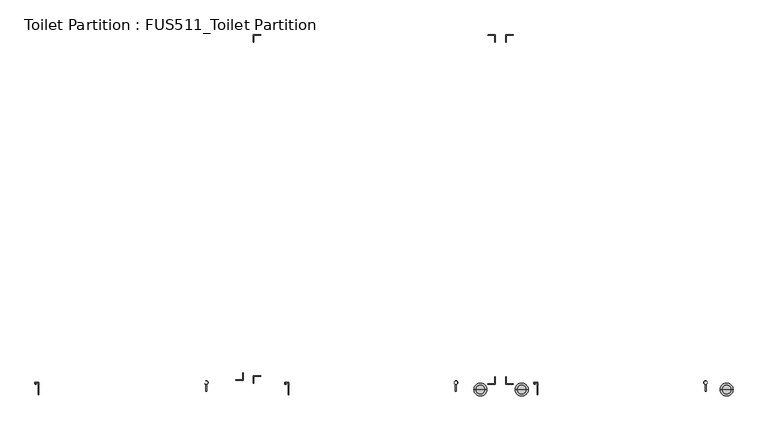
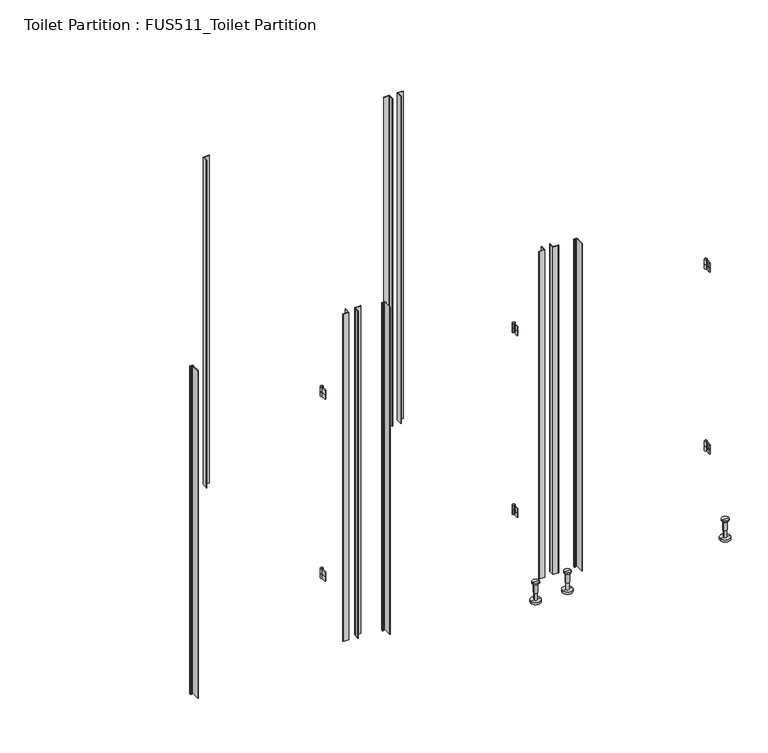
"""IFC4 building model written with IfcOpenShell, lengths in millimetres: furniture geometry, Toilet Partition : FUS511_Toilet Partition."""

import ifcopenshell
import ifcopenshell.guid

model = None  # the IFC model being written
_history = None  # IfcOwnerHistory: only IFC2X3 demands one
_inside = {}  # id of a spatial element -> (the spatial element, [elements in it])
_under = {}  # id of a project, library or spatial element -> (it, [spatial elements below it])
_declared = {}  # id of a project -> (the project, [libraries it declares])
_typed = {}  # id of a type object -> (the type object, [elements of that type])
_made_of = {}  # id of a material, layer set ... -> (it, [elements and type objects made of it])


def new_model(schema):
    """Start an empty IFC model of exactly this schema.

    Asked for "IFC4X3", IfcOpenShell would pick the latest addendum, in which some entities
    have other attributes; the version numbers below select the first issue.
    IFC2X3 requires an IfcOwnerHistory on every rooted entity: one is made here for all.
    """
    global model, _history
    if schema == "IFC4X3":
        model = ifcopenshell.file(schema_version=(4, 3, 0, 0))
    else:
        model = ifcopenshell.file(schema=schema)
    _inside.clear()
    _under.clear()
    _declared.clear()
    _typed.clear()
    _made_of.clear()
    _history = None
    if model.schema == "IFC2X3":
        org = make("IfcOrganization", Name="unknown")
        user = make(
            "IfcPersonAndOrganization",
            ThePerson=make("IfcPerson", FamilyName="unknown"),
            TheOrganization=org,
        )
        app = make(
            "IfcApplication",
            ApplicationDeveloper=org,
            Version="unknown",
            ApplicationFullName="unknown",
            ApplicationIdentifier="unknown",
        )
        _history = make(
            "IfcOwnerHistory",
            OwningUser=user,
            OwningApplication=app,
            ChangeAction="ADDED",
            CreationDate=0,
        )
    return model


def make(cls, **values):
    """One entity of the class cls with the attributes given. An attribute that is None is left unset."""
    return model.create_entity(
        cls, **{name: value for name, value in values.items() if value is not None}
    )


def rooted(cls, **values):
    """An entity with a GlobalId (a new one), such as an element, a storey or a relation."""
    return make(cls, GlobalId=ifcopenshell.guid.new(), OwnerHistory=_history, **values)


def si_unit(unit_type, name, prefix=None):
    """IfcSIUnit, for example si_unit("LENGTHUNIT", "METRE", prefix="MILLI")."""
    return make("IfcSIUnit", UnitType=unit_type, Prefix=prefix, Name=name)


def assignment(units):
    """IfcUnitAssignment: the units of a project."""
    return None if units is None else make("IfcUnitAssignment", Units=units)


def point(xyz):
    """IfcCartesianPoint."""
    return None if xyz is None else make("IfcCartesianPoint", Coordinates=xyz)


def direction(xyz):
    """IfcDirection."""
    return None if xyz is None else make("IfcDirection", DirectionRatios=xyz)


def frame(location, z_axis=None, x_axis=None):
    """IfcAxis2Placement3D, a coordinate frame: its origin and axes. An axis left out is left unset."""
    return make(
        "IfcAxis2Placement3D",
        Location=point(location),
        Axis=direction(z_axis),
        RefDirection=direction(x_axis),
    )


def frame_2d(location, x_axis=None):
    """IfcAxis2Placement2D, a coordinate frame in the plane: its origin and x axis."""
    return make(
        "IfcAxis2Placement2D", Location=point(location), RefDirection=direction(x_axis)
    )


def origin():
    """The frame at (0, 0, 0) with its axes left unset."""
    return frame((0.0, 0.0, 0.0))


def place(relative_to, where):
    """IfcLocalPlacement: puts the frame where relative to a parent placement (None: the world)."""
    return make(
        "IfcLocalPlacement", PlacementRelTo=relative_to, RelativePlacement=where
    )


def context(
    kind, dimensions, precision=None, world=None, true_north=None, identifier=None
):
    """IfcGeometricRepresentationContext, for example the 3D "Model" context."""
    return make(
        "IfcGeometricRepresentationContext",
        ContextIdentifier=identifier,
        ContextType=kind,
        CoordinateSpaceDimension=dimensions,
        Precision=precision,
        WorldCoordinateSystem=world,
        TrueNorth=true_north,
    )


def project(units=None, contexts=None):
    """IfcProject with its units and contexts."""
    return rooted(
        "IfcProject",
        Name="project",
        RepresentationContexts=contexts,
        UnitsInContext=assignment(units),
    )


def spatial(cls, under=None, at=None, **own):
    """A site, building, storey or space (cls), placed at a placement, below another one or the project."""
    s = rooted(cls, ObjectPlacement=at, **own)
    if under is not None:
        _under.setdefault(under.id(), (under, []))[1].append(s)
    return s


def polyline(points):
    """IfcPolyline through the points."""
    return make("IfcPolyline", Points=[point(p) for p in points])


def circle_curve(where, radius):
    """IfcCircle in the frame where."""
    return make("IfcCircle", Position=where, Radius=radius)


def trimmed(basis, trim1, trim2, sense, master):
    """IfcTrimmedCurve: the piece of a basis curve between two trims."""
    return make(
        "IfcTrimmedCurve",
        BasisCurve=basis,
        Trim1=trim1,
        Trim2=trim2,
        SenseAgreement=sense,
        MasterRepresentation=master,
    )


def segment(curve, same_sense, transition):
    """IfcCompositeCurveSegment."""
    return make(
        "IfcCompositeCurveSegment",
        Transition=transition,
        SameSense=same_sense,
        ParentCurve=curve,
    )


def composite_curve(segments, self_intersect=None):
    """IfcCompositeCurve: segments joined end to end."""
    return make("IfcCompositeCurve", Segments=segments, SelfIntersect=self_intersect)


def outline(outer, holes=None, kind="AREA"):
    """IfcArbitraryClosedProfileDef: a profile drawn as a closed curve; with holes, ...WithVoids."""
    if holes is None:
        return make("IfcArbitraryClosedProfileDef", ProfileType=kind, OuterCurve=outer)
    return make(
        "IfcArbitraryProfileDefWithVoids",
        ProfileType=kind,
        OuterCurve=outer,
        InnerCurves=holes,
    )


def extrude(swept, where, along, depth):
    """IfcExtrudedAreaSolid: the profile swept, set in the frame where, extruded along a direction by depth."""
    return make(
        "IfcExtrudedAreaSolid",
        SweptArea=swept,
        Position=where,
        ExtrudedDirection=direction(along),
        Depth=depth,
    )


def shape(context_of_items, identifier, shape_type, items):
    """IfcShapeRepresentation: the items that make up one representation, for example the "Body"."""
    return make(
        "IfcShapeRepresentation",
        ContextOfItems=context_of_items,
        RepresentationIdentifier=identifier,
        RepresentationType=shape_type,
        Items=items,
    )


def source(mapping_origin, context_of_items, identifier, shape_type, items):
    """IfcRepresentationMap: a shape defined once, which mapped items show again and again."""
    return make(
        "IfcRepresentationMap",
        MappingOrigin=mapping_origin,
        MappedRepresentation=shape(context_of_items, identifier, shape_type, items),
    )


def transform(
    local_origin,
    x_axis=None,
    y_axis=None,
    z_axis=None,
    scale=None,
    scale2=None,
    scale3=None,
    uniform=True,
):
    """IfcCartesianTransformationOperator3D, or its non-uniform kind. x_axis, y_axis, z_axis: its Axis1, 2, 3."""
    if uniform:
        return make(
            "IfcCartesianTransformationOperator3D",
            Axis1=direction(x_axis),
            Axis2=direction(y_axis),
            LocalOrigin=point(local_origin),
            Scale=scale,
            Axis3=direction(z_axis),
        )
    return make(
        "IfcCartesianTransformationOperator3DnonUniform",
        Axis1=direction(x_axis),
        Axis2=direction(y_axis),
        LocalOrigin=point(local_origin),
        Scale=scale,
        Axis3=direction(z_axis),
        Scale2=scale2,
        Scale3=scale3,
    )


def mapped(mapping_source, mapping_target):
    """IfcMappedItem: shows the shape of a source again, moved by a transform."""
    return make(
        "IfcMappedItem", MappingSource=mapping_source, MappingTarget=mapping_target
    )


def made_of(thing, what):
    """Note that an element or type object is made of a material, layer set ...; save() writes the relation."""
    if what is not None:
        _made_of.setdefault(what.id(), (what, []))[1].append(thing)
    return thing


def element(
    cls,
    number,
    at=None,
    inside=None,
    cuts=None,
    type_object=None,
    material=None,
    context=None,
    identifier="Body",
    shape_type=None,
    held_by="IfcProductDefinitionShape",
    body=None,
    shapes=None,
    **own,
):
    """One element of the class cls, such as IfcWall. Its Tag is "e" and its number.

    at: its placement. inside: the storey or other place that contains it. cuts: it is an
    opening in that element (IfcRelVoidsElement). A single representation is given by context,
    identifier, shape_type and body (its items); several are given by shapes. held_by: the class
    of the entity that holds the representations. save() writes the other relations.
    """
    e = rooted(cls, Tag="e%d" % number, ObjectPlacement=at, **own)
    if body is not None:
        shapes = [shape(context, identifier, shape_type, body)]
    if shapes is not None:
        e.Representation = make(held_by, Representations=shapes)
    if inside is not None:
        _inside.setdefault(inside.id(), (inside, []))[1].append(e)
    if cuts is not None:
        rooted(
            "IfcRelVoidsElement", RelatingBuildingElement=cuts, RelatedOpeningElement=e
        )
    if type_object is not None:
        _typed.setdefault(type_object.id(), (type_object, []))[1].append(e)
    return made_of(e, material)


def aggregate(whole, parts):
    """IfcRelAggregates: a whole, such as a stair, and the parts it consists of."""
    return rooted("IfcRelAggregates", RelatingObject=whole, RelatedObjects=parts)


def save(model, path):
    """Write the relations noted so far, then the file.

    IfcRelAggregates (storeys below a building ...), IfcRelContainedInSpatialStructure (elements
    in a storey), IfcRelDefinesByType, IfcRelAssociatesMaterial and IfcRelDeclares: one each for
    every whole, place, type object, material and project.
    """
    for whole, parts in _under.values():
        aggregate(whole, parts)
    for where, things in _inside.values():
        rooted(
            "IfcRelContainedInSpatialStructure",
            RelatedElements=things,
            RelatingStructure=where,
        )
    for kind, things in _typed.values():
        rooted("IfcRelDefinesByType", RelatedObjects=things, RelatingType=kind)
    for what, things in _made_of.values():
        rooted("IfcRelAssociatesMaterial", RelatedObjects=things, RelatingMaterial=what)
    for by, libraries in _declared.values():
        rooted("IfcRelDeclares", RelatingContext=by, RelatedDefinitions=libraries)
    model.write(path)


def plane_surface(at):
    """IfcPlane: the flat surface through the origin of the frame at, square to its z axis."""
    return make("IfcPlane", Position=at)


def cylinder_surface(at, radius):
    """IfcCylindricalSurface: all points at the distance radius from the z axis of the frame at."""
    return make("IfcCylindricalSurface", Position=at, Radius=radius)


def advanced_brep(points, edges, surfaces, faces):
    """IfcAdvancedBrep: a solid bounded by faces that lie on surfaces and meet in shared edges.

    An edge is (start, end): straight between two places in points (the first is 0);
    or (start, end, curve); or (start, end, curve, False) where it runs against its curve.
    A face is (place in surfaces, loops), or (place, loops, False) where it looks against
    its surface's normal. A loop lists edges by number (the first is 1), with a minus sign
    where the edge is run from its end to its start. The first loop is the outer one.
    """
    corners = [point(p) for p in points]
    vertices = [make("IfcVertexPoint", VertexGeometry=c) for c in corners]
    made = []
    for start, end, *more in edges:
        made.append(
            make(
                "IfcEdgeCurve",
                EdgeStart=vertices[start],
                EdgeEnd=vertices[end],
                EdgeGeometry=more[0] if more else make("IfcPolyline", Points=[corners[start], corners[end]]),
                SameSense=more[1] if len(more) > 1 else True,
            )
        )
    hull = []
    for where, loops, *sense in faces:
        bounds = []
        for j, loop in enumerate(loops):
            ring = [make("IfcOrientedEdge", EdgeElement=made[abs(k) - 1], Orientation=k > 0) for k in loop]
            bounds.append(
                make(
                    "IfcFaceOuterBound" if j == 0 else "IfcFaceBound",
                    Bound=make("IfcEdgeLoop", EdgeList=ring),
                    Orientation=True,
                )
            )
        hull.append(make("IfcAdvancedFace", Bounds=bounds, FaceSurface=surfaces[where], SameSense=sense[0] if sense else True))
    return make("IfcAdvancedBrep", Outer=make("IfcClosedShell", CfsFaces=hull))


def toilet_partition_fus511_toilet_partition_2a8fb3a8(model_context):
    return source(origin(), model_context, "Body", "SolidModel", [
        extrude(outline(composite_curve([segment(trimmed(circle_curve(frame_2d((-483.6851629, 1892.2118377)), 1.0008364), [point((-483.6851629, 1893.2126742))], [point((-484.6859993, 1892.2118377))], True, "CARTESIAN"), True, "CONTINUOUS"), segment(polyline([(-484.6859993, 1892.2118377), (-484.6859993, 1865.1892547), (-485.6868357, 1865.1892547)]), True, "CONTINUOUS"), segment(trimmed(circle_curve(frame_2d((-485.6868357, 1866.1900911)), 1.0008364), [point((-485.6868357, 1865.1892547))], [point((-486.6876721, 1866.1900911))], False, "CARTESIAN"), True, "CONTINUOUS"), segment(polyline([(-486.6876721, 1866.1900911), (-486.6876721, 1895.214347), (-457.6634163, 1895.214347)]), True, "CONTINUOUS"), segment(trimmed(circle_curve(frame_2d((-457.6634163, 1894.2135106)), 1.0008364), [point((-457.6634163, 1895.214347))], [point((-456.6625798, 1894.2135106))], False, "CARTESIAN"), True, "CONTINUOUS"), segment(polyline([(-456.6625798, 1894.2135106), (-456.6625798, 1893.2126742), (-483.6851629, 1893.2126742)]), True, "CONTINUOUS")], self_intersect=False)), frame((0.0, 0.0, 100.0), z_axis=(0.0, 0.0, 1.0), x_axis=(1.0, 0.0, 0.0)), (0.0, 0.0, 1.0), 1800.0),
        extrude(outline(composite_curve([segment(polyline([(478.8769058, 1893.2126742), (451.8543227, 1893.2126742), (451.8543227, 1894.2135106)]), True, "CONTINUOUS"), segment(trimmed(circle_curve(frame_2d((452.8551591, 1894.2135106)), 1.0008364), [point((451.8543227, 1894.2135106))], [point((452.8551591, 1895.214347))], False, "CARTESIAN"), True, "CONTINUOUS"), segment(polyline([(452.8551591, 1895.214347), (481.879415, 1895.214347), (481.879415, 1866.1900911)]), True, "CONTINUOUS"), segment(trimmed(circle_curve(frame_2d((480.8785786, 1866.1900911)), 1.0008364), [point((481.879415, 1866.1900911))], [point((480.8785786, 1865.1892547))], False, "CARTESIAN"), True, "CONTINUOUS"), segment(polyline([(480.8785786, 1865.1892547), (479.8777422, 1865.1892547), (479.8777422, 1892.2118377)]), True, "CONTINUOUS"), segment(trimmed(circle_curve(frame_2d((478.8769058, 1892.2118377)), 1.0008364), [point((479.8777422, 1892.2118377))], [point((478.8769058, 1893.2126742))], True, "CARTESIAN"), True, "CONTINUOUS")], self_intersect=False)), frame((0.0, 0.0, 100.0), z_axis=(0.0, 0.0, 1.0), x_axis=(1.0, 0.0, 0.0)), (0.0, 0.0, 1.0), 1800.0),
        extrude(outline(composite_curve([segment(trimmed(circle_curve(frame_2d((525.8819242, 1892.2118377)), 1.0008364), [point((525.8819242, 1893.2126742))], [point((524.8810878, 1892.2118377))], True, "CARTESIAN"), True, "CONTINUOUS"), segment(polyline([(524.8810878, 1892.2118377), (524.8810878, 1865.1892547), (523.8802514, 1865.1892547)]), True, "CONTINUOUS"), segment(trimmed(circle_curve(frame_2d((523.8802514, 1866.1900911)), 1.0008364), [point((523.8802514, 1865.1892547))], [point((522.879415, 1866.1900911))], False, "CARTESIAN"), True, "CONTINUOUS"), segment(polyline([(522.879415, 1866.1900911), (522.879415, 1895.214347), (551.9036709, 1895.214347)]), True, "CONTINUOUS"), segment(trimmed(circle_curve(frame_2d((551.9036709, 1894.2135106)), 1.0008364), [point((551.9036709, 1895.214347))], [point((552.9045073, 1894.2135106))], False, "CARTESIAN"), True, "CONTINUOUS"), segment(polyline([(552.9045073, 1894.2135106), (552.9045073, 1893.2126742), (525.8819242, 1893.2126742)]), True, "CONTINUOUS")], self_intersect=False)), frame((0.0, 0.0, 100.0), z_axis=(0.0, 0.0, 1.0), x_axis=(1.0, 0.0, 0.0)), (0.0, 0.0, 1.0), 1800.0),
        extrude(outline(composite_curve([segment(trimmed(circle_curve(frame_2d((-530.6901814, 514.4572016)), 1.0008364), [point((-530.6901814, 513.4563652))], [point((-529.689345, 514.4572016))], True, "CARTESIAN"), True, "CONTINUOUS"), segment(polyline([(-529.689345, 514.4572016), (-529.689345, 541.4797847), (-528.6885085, 541.4797847)]), True, "CONTINUOUS"), segment(trimmed(circle_curve(frame_2d((-528.6885085, 540.4789483)), 1.0008364), [point((-528.6885085, 541.4797847))], [point((-527.6876721, 540.4789483))], False, "CARTESIAN"), True, "CONTINUOUS"), segment(polyline([(-527.6876721, 540.4789483), (-527.6876721, 511.4546924), (-556.711928, 511.4546924)]), True, "CONTINUOUS"), segment(trimmed(circle_curve(frame_2d((-556.711928, 512.4555288)), 1.0008364), [point((-556.711928, 511.4546924))], [point((-557.7127644, 512.4555288))], False, "CARTESIAN"), True, "CONTINUOUS"), segment(polyline([(-557.7127644, 512.4555288), (-557.7127644, 513.4563652), (-530.6901814, 513.4563652)]), True, "CONTINUOUS")], self_intersect=False)), frame((0.0, 0.0, 100.0), z_axis=(0.0, 0.0, 1.0), x_axis=(1.0, 0.0, 0.0)), (0.0, 0.0, 1.0), 1800.0),
        extrude(outline(composite_curve([segment(trimmed(circle_curve(frame_2d((-483.6851629, 527.0159753)), 1.0008364), [point((-483.6851629, 528.0168117))], [point((-484.6859993, 527.0159753))], True, "CARTESIAN"), True, "CONTINUOUS"), segment(polyline([(-484.6859993, 527.0159753), (-484.6859993, 499.9933923), (-485.6868357, 499.9933923)]), True, "CONTINUOUS"), segment(trimmed(circle_curve(frame_2d((-485.6868357, 500.9942287)), 1.0008364), [point((-485.6868357, 499.9933923))], [point((-486.6876721, 500.9942287))], False, "CARTESIAN"), True, "CONTINUOUS"), segment(polyline([(-486.6876721, 500.9942287), (-486.6876721, 530.0184846), (-457.6634163, 530.0184846)]), True, "CONTINUOUS"), segment(trimmed(circle_curve(frame_2d((-457.6634163, 529.0176481)), 1.0008364), [point((-457.6634163, 530.0184846))], [point((-456.6625798, 529.0176481))], False, "CARTESIAN"), True, "CONTINUOUS"), segment(polyline([(-456.6625798, 529.0176481), (-456.6625798, 528.0168117), (-483.6851629, 528.0168117)]), True, "CONTINUOUS")], self_intersect=False)), frame((0.0, 0.0, 100.0), z_axis=(0.0, 0.0, 1.0), x_axis=(1.0, 0.0, 0.0)), (0.0, 0.0, 1.0), 1800.0),
        extrude(outline(composite_curve([segment(trimmed(circle_curve(frame_2d((478.8769058, 498.2168562)), 1.0008364), [point((478.8769058, 497.2160198))], [point((479.8777422, 498.2168562))], True, "CARTESIAN"), True, "CONTINUOUS"), segment(polyline([(479.8777422, 498.2168562), (479.8777422, 525.2394393), (480.8785786, 525.2394393)]), True, "CONTINUOUS"), segment(trimmed(circle_curve(frame_2d((480.8785786, 524.2386029)), 1.0008364), [point((480.8785786, 525.2394393))], [point((481.879415, 524.2386029))], False, "CARTESIAN"), True, "CONTINUOUS"), segment(polyline([(481.879415, 524.2386029), (481.879415, 495.214347), (452.8551591, 495.214347)]), True, "CONTINUOUS"), segment(trimmed(circle_curve(frame_2d((452.8551591, 496.2151834)), 1.0008364), [point((452.8551591, 495.214347))], [point((451.8543227, 496.2151834))], False, "CARTESIAN"), True, "CONTINUOUS"), segment(polyline([(451.8543227, 496.2151834), (451.8543227, 497.2160198), (478.8769058, 497.2160198)]), True, "CONTINUOUS")], self_intersect=False)), frame((0.0, 0.0, 100.0), z_axis=(0.0, 0.0, 1.0), x_axis=(1.0, 0.0, 0.0)), (0.0, 0.0, 1.0), 1800.0),
        extrude(outline(composite_curve([segment(polyline([(525.8819242, 497.2160198), (552.9045073, 497.2160198), (552.9045073, 496.2151834)]), True, "CONTINUOUS"), segment(trimmed(circle_curve(frame_2d((551.9036709, 496.2151834)), 1.0008364), [point((552.9045073, 496.2151834))], [point((551.9036709, 495.214347))], False, "CARTESIAN"), True, "CONTINUOUS"), segment(polyline([(551.9036709, 495.214347), (522.879415, 495.214347), (522.879415, 524.2386029)]), True, "CONTINUOUS"), segment(trimmed(circle_curve(frame_2d((523.8802514, 524.2386029)), 1.0008364), [point((522.879415, 524.2386029))], [point((523.8802514, 525.2394393))], False, "CARTESIAN"), True, "CONTINUOUS"), segment(polyline([(523.8802514, 525.2394393), (524.8810878, 525.2394393), (524.8810878, 498.2168562)]), True, "CONTINUOUS"), segment(trimmed(circle_curve(frame_2d((525.8819242, 498.2168562)), 1.0008364), [point((524.8810878, 498.2168562))], [point((525.8819242, 497.2160198))], True, "CARTESIAN"), True, "CONTINUOUS")], self_intersect=False)), frame((0.0, 0.0, 100.0), z_axis=(0.0, 0.0, 1.0), x_axis=(1.0, 0.0, 0.0)), (0.0, 0.0, 1.0), 1800.0),
        extrude(outline(composite_curve([segment(trimmed(circle_curve(frame_2d((1322.6156791, 502.2850056)), 7.0), [point((1320.6156791, 495.5768017))], [point((1324.6156791, 495.5768017))], False, "CARTESIAN"), True, "CONTINUOUS"), segment(polyline([(1324.6156791, 495.5768017), (1324.6156791, 467.7850056), (1320.6156791, 467.7850056), (1320.6156791, 495.5768017)]), True, "CONTINUOUS")], self_intersect=False), holes=[composite_curve([segment(trimmed(circle_curve(frame_2d((1322.6156791, 502.2850056)), 6.0), [point((1316.6156791, 502.2850056))], [point((1328.6156791, 502.2850056))], True, "CARTESIAN"), True, "CONTINUOUS"), segment(trimmed(circle_curve(frame_2d((1322.6156791, 502.2850056)), 6.0), [point((1328.6156791, 502.2850056))], [point((1316.6156791, 502.2850056))], True, "CARTESIAN"), True, "CONTINUOUS")], self_intersect=False)]), frame((0.0, 0.0, 1525.0), z_axis=(0.0, 0.0, 1.0), x_axis=(1.0, 0.0, 0.0)), (0.0, 0.0, 1.0), 25.0),
        extrude(outline(composite_curve([segment(trimmed(circle_curve(frame_2d((1322.6156791, 502.2850056)), 7.0), [point((1320.6156791, 495.5768017))], [point((1324.6156791, 495.5768017))], False, "CARTESIAN"), True, "CONTINUOUS"), segment(polyline([(1324.6156791, 495.5768017), (1324.6156791, 467.7850056), (1320.6156791, 467.7850056), (1320.6156791, 495.5768017)]), True, "CONTINUOUS")], self_intersect=False), holes=[composite_curve([segment(trimmed(circle_curve(frame_2d((1322.6156791, 502.2850056)), 6.0), [point((1316.6156791, 502.2850056))], [point((1328.6156791, 502.2850056))], True, "CARTESIAN"), True, "CONTINUOUS"), segment(trimmed(circle_curve(frame_2d((1322.6156791, 502.2850056)), 6.0), [point((1328.6156791, 502.2850056))], [point((1316.6156791, 502.2850056))], True, "CARTESIAN"), True, "CONTINUOUS")], self_intersect=False)]), frame((0.0, 0.0, 1500.0), z_axis=(0.0, 0.0, 1.0), x_axis=(1.0, 0.0, 0.0)), (0.0, 0.0, 1.0), 25.0),
        extrude(outline(composite_curve([segment(trimmed(circle_curve(frame_2d((323.7360042, 502.2850056)), 7.0), [point((321.7360042, 495.5768017))], [point((325.7360042, 495.5768017))], False, "CARTESIAN"), True, "CONTINUOUS"), segment(polyline([(325.7360042, 495.5768017), (325.7360042, 467.7850056), (321.7360042, 467.7850056), (321.7360042, 495.5768017)]), True, "CONTINUOUS")], self_intersect=False), holes=[composite_curve([segment(trimmed(circle_curve(frame_2d((323.7360042, 502.2850056)), 6.0), [point((317.7360042, 502.2850056))], [point((329.7360042, 502.2850056))], True, "CARTESIAN"), True, "CONTINUOUS"), segment(trimmed(circle_curve(frame_2d((323.7360042, 502.2850056)), 6.0), [point((329.7360042, 502.2850056))], [point((317.7360042, 502.2850056))], True, "CARTESIAN"), True, "CONTINUOUS")], self_intersect=False)]), frame((0.0, 0.0, 1525.0), z_axis=(0.0, 0.0, 1.0), x_axis=(1.0, 0.0, 0.0)), (0.0, 0.0, 1.0), 25.0),
        extrude(outline(composite_curve([segment(trimmed(circle_curve(frame_2d((323.7360042, 502.2850056)), 7.0), [point((321.7360042, 495.5768017))], [point((325.7360042, 495.5768017))], False, "CARTESIAN"), True, "CONTINUOUS"), segment(polyline([(325.7360042, 495.5768017), (325.7360042, 467.7850056), (321.7360042, 467.7850056), (321.7360042, 495.5768017)]), True, "CONTINUOUS")], self_intersect=False), holes=[composite_curve([segment(trimmed(circle_curve(frame_2d((323.7360042, 502.2850056)), 6.0), [point((317.7360042, 502.2850056))], [point((329.7360042, 502.2850056))], True, "CARTESIAN"), True, "CONTINUOUS"), segment(trimmed(circle_curve(frame_2d((323.7360042, 502.2850056)), 6.0), [point((329.7360042, 502.2850056))], [point((317.7360042, 502.2850056))], True, "CARTESIAN"), True, "CONTINUOUS")], self_intersect=False)]), frame((0.0, 0.0, 1500.0), z_axis=(0.0, 0.0, 1.0), x_axis=(1.0, 0.0, 0.0)), (0.0, 0.0, 1.0), 25.0),
        extrude(outline(composite_curve([segment(trimmed(circle_curve(frame_2d((-675.1953266, 502.2850056)), 7.0), [point((-677.1953266, 495.5768017))], [point((-673.1953266, 495.5768017))], False, "CARTESIAN"), True, "CONTINUOUS"), segment(polyline([(-673.1953266, 495.5768017), (-673.1953266, 467.7850056), (-677.1953266, 467.7850056), (-677.1953266, 495.5768017)]), True, "CONTINUOUS")], self_intersect=False), holes=[composite_curve([segment(trimmed(circle_curve(frame_2d((-675.1953266, 502.2850056)), 6.0), [point((-681.1953266, 502.2850056))], [point((-669.1953266, 502.2850056))], True, "CARTESIAN"), True, "CONTINUOUS"), segment(trimmed(circle_curve(frame_2d((-675.1953266, 502.2850056)), 6.0), [point((-669.1953266, 502.2850056))], [point((-681.1953266, 502.2850056))], True, "CARTESIAN"), True, "CONTINUOUS")], self_intersect=False)]), frame((0.0, 0.0, 1525.0), z_axis=(0.0, 0.0, 1.0), x_axis=(1.0, 0.0, 0.0)), (0.0, 0.0, 1.0), 25.0),
        extrude(outline(composite_curve([segment(trimmed(circle_curve(frame_2d((-675.1953266, 502.2850056)), 7.0), [point((-677.1953266, 495.5768017))], [point((-673.1953266, 495.5768017))], False, "CARTESIAN"), True, "CONTINUOUS"), segment(polyline([(-673.1953266, 495.5768017), (-673.1953266, 467.7850056), (-677.1953266, 467.7850056), (-677.1953266, 495.5768017)]), True, "CONTINUOUS")], self_intersect=False), holes=[composite_curve([segment(trimmed(circle_curve(frame_2d((-675.1953266, 502.2850056)), 6.0), [point((-681.1953266, 502.2850056))], [point((-669.1953266, 502.2850056))], True, "CARTESIAN"), True, "CONTINUOUS"), segment(trimmed(circle_curve(frame_2d((-675.1953266, 502.2850056)), 6.0), [point((-669.1953266, 502.2850056))], [point((-681.1953266, 502.2850056))], True, "CARTESIAN"), True, "CONTINUOUS")], self_intersect=False)]), frame((0.0, 0.0, 1500.0), z_axis=(0.0, 0.0, 1.0), x_axis=(1.0, 0.0, 0.0)), (0.0, 0.0, 1.0), 25.0),
        extrude(outline(composite_curve([segment(trimmed(circle_curve(frame_2d((1322.6156791, 502.2850056)), 7.0), [point((1320.6156791, 495.5768017))], [point((1324.6156791, 495.5768017))], False, "CARTESIAN"), True, "CONTINUOUS"), segment(polyline([(1324.6156791, 495.5768017), (1324.6156791, 467.7850056), (1320.6156791, 467.7850056), (1320.6156791, 495.5768017)]), True, "CONTINUOUS")], self_intersect=False), holes=[composite_curve([segment(trimmed(circle_curve(frame_2d((1322.6156791, 502.2850056)), 6.0), [point((1316.6156791, 502.2850056))], [point((1328.6156791, 502.2850056))], True, "CARTESIAN"), True, "CONTINUOUS"), segment(trimmed(circle_curve(frame_2d((1322.6156791, 502.2850056)), 6.0), [point((1328.6156791, 502.2850056))], [point((1316.6156791, 502.2850056))], True, "CARTESIAN"), True, "CONTINUOUS")], self_intersect=False)]), frame((0.0, 0.0, 525.0), z_axis=(0.0, 0.0, 1.0), x_axis=(1.0, 0.0, 0.0)), (0.0, 0.0, 1.0), 25.0),
        extrude(outline(composite_curve([segment(trimmed(circle_curve(frame_2d((1322.6156791, 502.2850056)), 7.0), [point((1320.6156791, 495.5768017))], [point((1324.6156791, 495.5768017))], False, "CARTESIAN"), True, "CONTINUOUS"), segment(polyline([(1324.6156791, 495.5768017), (1324.6156791, 467.7850056), (1320.6156791, 467.7850056), (1320.6156791, 495.5768017)]), True, "CONTINUOUS")], self_intersect=False), holes=[composite_curve([segment(trimmed(circle_curve(frame_2d((1322.6156791, 502.2850056)), 6.0), [point((1316.6156791, 502.2850056))], [point((1328.6156791, 502.2850056))], True, "CARTESIAN"), True, "CONTINUOUS"), segment(trimmed(circle_curve(frame_2d((1322.6156791, 502.2850056)), 6.0), [point((1328.6156791, 502.2850056))], [point((1316.6156791, 502.2850056))], True, "CARTESIAN"), True, "CONTINUOUS")], self_intersect=False)]), frame((0.0, 0.0, 500.0), z_axis=(0.0, 0.0, 1.0), x_axis=(1.0, 0.0, 0.0)), (0.0, 0.0, 1.0), 25.0),
        extrude(outline(composite_curve([segment(trimmed(circle_curve(frame_2d((323.7360042, 502.2850056)), 7.0), [point((321.7360042, 495.5768017))], [point((325.7360042, 495.5768017))], False, "CARTESIAN"), True, "CONTINUOUS"), segment(polyline([(325.7360042, 495.5768017), (325.7360042, 467.7850056), (321.7360042, 467.7850056), (321.7360042, 495.5768017)]), True, "CONTINUOUS")], self_intersect=False), holes=[composite_curve([segment(trimmed(circle_curve(frame_2d((323.7360042, 502.2850056)), 6.0), [point((317.7360042, 502.2850056))], [point((329.7360042, 502.2850056))], True, "CARTESIAN"), True, "CONTINUOUS"), segment(trimmed(circle_curve(frame_2d((323.7360042, 502.2850056)), 6.0), [point((329.7360042, 502.2850056))], [point((317.7360042, 502.2850056))], True, "CARTESIAN"), True, "CONTINUOUS")], self_intersect=False)]), frame((0.0, 0.0, 525.0), z_axis=(0.0, 0.0, 1.0), x_axis=(1.0, 0.0, 0.0)), (0.0, 0.0, 1.0), 25.0),
        extrude(outline(composite_curve([segment(trimmed(circle_curve(frame_2d((323.7360042, 502.2850056)), 7.0), [point((321.7360042, 495.5768017))], [point((325.7360042, 495.5768017))], False, "CARTESIAN"), True, "CONTINUOUS"), segment(polyline([(325.7360042, 495.5768017), (325.7360042, 467.7850056), (321.7360042, 467.7850056), (321.7360042, 495.5768017)]), True, "CONTINUOUS")], self_intersect=False), holes=[composite_curve([segment(trimmed(circle_curve(frame_2d((323.7360042, 502.2850056)), 6.0), [point((317.7360042, 502.2850056))], [point((329.7360042, 502.2850056))], True, "CARTESIAN"), True, "CONTINUOUS"), segment(trimmed(circle_curve(frame_2d((323.7360042, 502.2850056)), 6.0), [point((329.7360042, 502.2850056))], [point((317.7360042, 502.2850056))], True, "CARTESIAN"), True, "CONTINUOUS")], self_intersect=False)]), frame((0.0, 0.0, 500.0), z_axis=(0.0, 0.0, 1.0), x_axis=(1.0, 0.0, 0.0)), (0.0, 0.0, 1.0), 25.0),
        extrude(outline(composite_curve([segment(trimmed(circle_curve(frame_2d((-675.1953266, 502.2850056)), 7.0), [point((-677.1953266, 495.5768017))], [point((-673.1953266, 495.5768017))], False, "CARTESIAN"), True, "CONTINUOUS"), segment(polyline([(-673.1953266, 495.5768017), (-673.1953266, 467.7850056), (-677.1953266, 467.7850056), (-677.1953266, 495.5768017)]), True, "CONTINUOUS")], self_intersect=False), holes=[composite_curve([segment(trimmed(circle_curve(frame_2d((-675.1953266, 502.2850056)), 6.0), [point((-681.1953266, 502.2850056))], [point((-669.1953266, 502.2850056))], True, "CARTESIAN"), True, "CONTINUOUS"), segment(trimmed(circle_curve(frame_2d((-675.1953266, 502.2850056)), 6.0), [point((-669.1953266, 502.2850056))], [point((-681.1953266, 502.2850056))], True, "CARTESIAN"), True, "CONTINUOUS")], self_intersect=False)]), frame((0.0, 0.0, 525.0), z_axis=(0.0, 0.0, 1.0), x_axis=(1.0, 0.0, 0.0)), (0.0, 0.0, 1.0), 25.0),
        extrude(outline(composite_curve([segment(trimmed(circle_curve(frame_2d((-675.1953266, 502.2850056)), 7.0), [point((-677.1953266, 495.5768017))], [point((-673.1953266, 495.5768017))], False, "CARTESIAN"), True, "CONTINUOUS"), segment(polyline([(-673.1953266, 495.5768017), (-673.1953266, 467.7850056), (-677.1953266, 467.7850056), (-677.1953266, 495.5768017)]), True, "CONTINUOUS")], self_intersect=False), holes=[composite_curve([segment(trimmed(circle_curve(frame_2d((-675.1953266, 502.2850056)), 6.0), [point((-681.1953266, 502.2850056))], [point((-669.1953266, 502.2850056))], True, "CARTESIAN"), True, "CONTINUOUS"), segment(trimmed(circle_curve(frame_2d((-675.1953266, 502.2850056)), 6.0), [point((-669.1953266, 502.2850056))], [point((-681.1953266, 502.2850056))], True, "CARTESIAN"), True, "CONTINUOUS")], self_intersect=False)]), frame((0.0, 0.0, 500.0), z_axis=(0.0, 0.0, 1.0), x_axis=(1.0, 0.0, 0.0)), (0.0, 0.0, 1.0), 25.0),
        extrude(outline(polyline([(635.6294456, 503.4888254), (651.4228263, 503.4888254), (651.4228263, 499.4012527), (653.8741408, 495.1554513), (652.7343518, 495.1554513), (651.4228263, 497.4270801), (651.4228263, 454.1345106), (649.4486537, 454.1345106), (649.4486537, 501.5146528), (645.826099, 501.5146528), (641.7674724, 497.0112968), (640.6276833, 497.0112968), (644.6863099, 501.5146528), (636.6165319, 501.5146528), (636.6165319, 497.8847941), (638.0262016, 497.8847941), (638.0262016, 497.0402783), (635.6294456, 497.0402783), (635.6294456, 503.4888254)])), frame((0.0, 0.0, 100.0), z_axis=(0.0, 0.0, 1.0), x_axis=(1.0, 0.0, 0.0)), (0.0, 0.0, 1.0), 1800.0),
        extrude(outline(composite_curve([segment(polyline([(640.8337808, 495.214347), (637.7985331, 495.214347)]), True, "CONTINUOUS"), segment(trimmed(circle_curve(frame_2d((637.7985331, 496.004016)), 0.789669), [point((637.7985331, 495.214347))], [point((637.0088641, 496.004016))], False, "CARTESIAN"), True, "CONTINUOUS"), segment(polyline([(637.0088641, 496.004016), (637.0088641, 496.8402783), (638.1566952, 496.8402783)]), True, "CONTINUOUS"), segment(trimmed(circle_curve(frame_2d((637.5137871, 497.4916495)), 0.9152132), [point((638.1566952, 496.8402783))], [point((638.1251074, 498.1727534))], True, "CARTESIAN"), True, "CONTINUOUS"), segment(trimmed(circle_curve(frame_2d((638.4034381, 498.4828563)), 0.4166915), [point((638.1251074, 498.1727534))], [point((638.2496827, 498.870143))], False, "CARTESIAN"), True, "CONTINUOUS"), segment(trimmed(circle_curve(frame_2d((639.3215602, 496.1702449)), 2.9048875), [point((638.2496827, 498.870143))], [point((640.4174512, 498.8604854))], False, "CARTESIAN"), True, "CONTINUOUS"), segment(trimmed(circle_curve(frame_2d((640.2672492, 498.4917631)), 0.3981417), [point((640.4174512, 498.8604854))], [point((640.5253128, 498.1885801))], False, "CARTESIAN"), True, "CONTINUOUS"), segment(trimmed(circle_curve(frame_2d((641.1185268, 497.4916495)), 0.9152132), [point((640.5253128, 498.1885801))], [point((640.4756187, 496.8402783))], True, "CARTESIAN"), True, "CONTINUOUS"), segment(polyline([(640.4756187, 496.8402783), (641.6234499, 496.8402783), (641.6234499, 496.004016)]), True, "CONTINUOUS"), segment(trimmed(circle_curve(frame_2d((640.8337808, 496.004016)), 0.789669), [point((641.6234499, 496.004016))], [point((640.8337808, 495.214347))], False, "CARTESIAN"), True, "CONTINUOUS")], self_intersect=False)), frame((0.0, 0.0, 100.0), z_axis=(0.0, 0.0, 1.0), x_axis=(1.0, 0.0, 0.0)), (0.0, 0.0, 1.0), 1800.0),
        extrude(outline(polyline([(-362.0057179, 503.4888254), (-346.2123372, 503.4888254), (-346.2123372, 499.4012527), (-343.7610226, 495.1554513), (-344.9008117, 495.1554513), (-346.2123372, 497.4270801), (-346.2123372, 454.1345106), (-348.1865098, 454.1345106), (-348.1865098, 501.5146528), (-351.8090644, 501.5146528), (-355.8676911, 497.0112968), (-357.0074802, 497.0112968), (-352.9488535, 501.5146528), (-361.0186316, 501.5146528), (-361.0186316, 497.8847941), (-359.6089619, 497.8847941), (-359.6089619, 497.0402783), (-362.0057179, 497.0402783), (-362.0057179, 503.4888254)])), frame((0.0, 0.0, 100.0), z_axis=(0.0, 0.0, 1.0), x_axis=(1.0, 0.0, 0.0)), (0.0, 0.0, 1.0), 1800.0),
        extrude(outline(composite_curve([segment(polyline([(-356.8013826, 495.214347), (-359.8366303, 495.214347)]), True, "CONTINUOUS"), segment(trimmed(circle_curve(frame_2d((-359.8366303, 496.004016)), 0.789669), [point((-359.8366303, 495.214347))], [point((-360.6262994, 496.004016))], False, "CARTESIAN"), True, "CONTINUOUS"), segment(polyline([(-360.6262994, 496.004016), (-360.6262994, 496.8402783), (-359.4784683, 496.8402783)]), True, "CONTINUOUS"), segment(trimmed(circle_curve(frame_2d((-360.1213764, 497.4916495)), 0.9152132), [point((-359.4784683, 496.8402783))], [point((-359.510056, 498.1727534))], True, "CARTESIAN"), True, "CONTINUOUS"), segment(trimmed(circle_curve(frame_2d((-359.2317253, 498.4828563)), 0.4166915), [point((-359.510056, 498.1727534))], [point((-359.3854807, 498.870143))], False, "CARTESIAN"), True, "CONTINUOUS"), segment(trimmed(circle_curve(frame_2d((-358.3136033, 496.1702449)), 2.9048875), [point((-359.3854807, 498.870143))], [point((-357.2177122, 498.8604854))], False, "CARTESIAN"), True, "CONTINUOUS"), segment(trimmed(circle_curve(frame_2d((-357.3679142, 498.4917631)), 0.3981417), [point((-357.2177122, 498.8604854))], [point((-357.1098506, 498.1885801))], False, "CARTESIAN"), True, "CONTINUOUS"), segment(trimmed(circle_curve(frame_2d((-356.5166366, 497.4916495)), 0.9152132), [point((-357.1098506, 498.1885801))], [point((-357.1595447, 496.8402783))], True, "CARTESIAN"), True, "CONTINUOUS"), segment(polyline([(-357.1595447, 496.8402783), (-356.0117136, 496.8402783), (-356.0117136, 496.004016)]), True, "CONTINUOUS"), segment(trimmed(circle_curve(frame_2d((-356.8013826, 496.004016)), 0.789669), [point((-356.0117136, 496.004016))], [point((-356.8013826, 495.214347))], False, "CARTESIAN"), True, "CONTINUOUS")], self_intersect=False)), frame((0.0, 0.0, 100.0), z_axis=(0.0, 0.0, 1.0), x_axis=(1.0, 0.0, 0.0)), (0.0, 0.0, 1.0), 1800.0),
        extrude(outline(polyline([(-1360.9370525, 503.4888254), (-1345.1436718, 503.4888254), (-1345.1436718, 499.4012527), (-1342.6923572, 495.1554513), (-1343.8321463, 495.1554513), (-1345.1436718, 497.4270801), (-1345.1436718, 454.1345106), (-1347.1178444, 454.1345106), (-1347.1178444, 501.5146528), (-1350.740399, 501.5146528), (-1354.7990257, 497.0112968), (-1355.9388148, 497.0112968), (-1351.8801881, 501.5146528), (-1359.9499662, 501.5146528), (-1359.9499662, 497.8847941), (-1358.5402965, 497.8847941), (-1358.5402965, 497.0402783), (-1360.9370525, 497.0402783), (-1360.9370525, 503.4888254)])), frame((0.0, 0.0, 100.0), z_axis=(0.0, 0.0, 1.0), x_axis=(1.0, 0.0, 0.0)), (0.0, 0.0, 1.0), 1800.0),
        extrude(outline(composite_curve([segment(polyline([(-1355.7327172, 495.214347), (-1358.7679649, 495.214347)]), True, "CONTINUOUS"), segment(trimmed(circle_curve(frame_2d((-1358.7679649, 496.004016)), 0.789669), [point((-1358.7679649, 495.214347))], [point((-1359.557634, 496.004016))], False, "CARTESIAN"), True, "CONTINUOUS"), segment(polyline([(-1359.557634, 496.004016), (-1359.557634, 496.8402783), (-1358.4098029, 496.8402783)]), True, "CONTINUOUS"), segment(trimmed(circle_curve(frame_2d((-1359.052711, 497.4916495)), 0.9152132), [point((-1358.4098029, 496.8402783))], [point((-1358.4413906, 498.1727534))], True, "CARTESIAN"), True, "CONTINUOUS"), segment(trimmed(circle_curve(frame_2d((-1358.1630599, 498.4828563)), 0.4166915), [point((-1358.4413906, 498.1727534))], [point((-1358.3168153, 498.870143))], False, "CARTESIAN"), True, "CONTINUOUS"), segment(trimmed(circle_curve(frame_2d((-1357.2449378, 496.1702449)), 2.9048875), [point((-1358.3168153, 498.870143))], [point((-1356.1490468, 498.8604854))], False, "CARTESIAN"), True, "CONTINUOUS"), segment(trimmed(circle_curve(frame_2d((-1356.2992488, 498.4917631)), 0.3981417), [point((-1356.1490468, 498.8604854))], [point((-1356.0411852, 498.1885801))], False, "CARTESIAN"), True, "CONTINUOUS"), segment(trimmed(circle_curve(frame_2d((-1355.4479712, 497.4916495)), 0.9152132), [point((-1356.0411852, 498.1885801))], [point((-1356.0908793, 496.8402783))], True, "CARTESIAN"), True, "CONTINUOUS"), segment(polyline([(-1356.0908793, 496.8402783), (-1354.9430482, 496.8402783), (-1354.9430482, 496.004016)]), True, "CONTINUOUS"), segment(trimmed(circle_curve(frame_2d((-1355.7327172, 496.004016)), 0.789669), [point((-1354.9430482, 496.004016))], [point((-1355.7327172, 495.214347))], False, "CARTESIAN"), True, "CONTINUOUS")], self_intersect=False)), frame((0.0, 0.0, 100.0), z_axis=(0.0, 0.0, 1.0), x_axis=(1.0, 0.0, 0.0)), (0.0, 0.0, 1.0), 1800.0),
        advanced_brep(
        [(1391.087395, 474.714347, 104.1461397), (1422.3312369, 474.714347, 104.1461397), (1422.3312369, 474.714347, 101.0217555), (1391.087395, 474.714347, 101.0217555), (1380.6727811, 474.714347, 0.0), (1432.7458509, 474.714347, 0.0), (1406.709316, 474.714347, 0.0), (1380.6727811, 474.714347, 10.414614), (1432.7458509, 474.714347, 10.414614), (1398.8983555, 474.714347, 10.414614), (1414.5202765, 474.714347, 10.414614), (1398.8983555, 474.714347, 52.0730698), (1414.5202765, 474.714347, 52.0730698), (1396.294702, 474.714347, 52.0730698), (1417.1239299, 474.714347, 52.0730698), (1396.294702, 474.714347, 101.0217555), (1417.1239299, 474.714347, 101.0217555), (1389.0044722, 474.714347, 104.1461397), (1424.4141597, 474.714347, 104.1461397), (1389.0044722, 474.714347, 110.394908), (1424.4141597, 474.714347, 110.394908), (1406.709316, 474.714347, 110.394908)],
        [
            (0, 1, circle_curve(frame((1406.709316, 474.714347, 104.1461397), z_axis=(0.0, 0.0, -1.0), x_axis=(1.0, 0.0, 0.0)), 15.6219209)),
            (1, 2),
            (2, 3, circle_curve(frame((1406.709316, 474.714347, 101.0217555), z_axis=(0.0, 0.0, 1.0), x_axis=(1.0, 0.0, 0.0)), 15.6219209)),
            (3, 0),
            (1, 0, circle_curve(frame((1406.709316, 474.714347, 104.1461397), z_axis=(0.0, 0.0, -1.0), x_axis=(1.0, 0.0, 0.0)), 15.6219209)),
            (3, 2, circle_curve(frame((1406.709316, 474.714347, 101.0217555), z_axis=(0.0, 0.0, 1.0), x_axis=(1.0, 0.0, 0.0)), 15.6219209)),
            (4, 5, circle_curve(frame((1406.709316, 474.714347, 0.0), z_axis=(0.0, 0.0, -1.0), x_axis=(1.0, 0.0, 0.0)), 26.0365349)),
            (5, 6),
            (6, 4),
            (5, 4, circle_curve(frame((1406.709316, 474.714347, 0.0), z_axis=(0.0, 0.0, -1.0), x_axis=(1.0, 0.0, 0.0)), 26.0365349)),
            (7, 8, circle_curve(frame((1406.709316, 474.714347, 10.414614), z_axis=(0.0, 0.0, -1.0), x_axis=(1.0, 0.0, 0.0)), 26.0365349)),
            (8, 5),
            (4, 7),
            (8, 7, circle_curve(frame((1406.709316, 474.714347, 10.414614), z_axis=(0.0, 0.0, -1.0), x_axis=(1.0, 0.0, 0.0)), 26.0365349)),
            (9, 10, circle_curve(frame((1406.709316, 474.714347, 10.414614), z_axis=(0.0, 0.0, -1.0), x_axis=(1.0, 0.0, 0.0)), 7.8109605)),
            (10, 8),
            (7, 9),
            (10, 9, circle_curve(frame((1406.709316, 474.714347, 10.414614), z_axis=(0.0, 0.0, -1.0), x_axis=(1.0, 0.0, 0.0)), 7.8109605)),
            (11, 12, circle_curve(frame((1406.709316, 474.714347, 52.0730698), z_axis=(0.0, 0.0, -1.0), x_axis=(1.0, 0.0, 0.0)), 7.8109605)),
            (12, 10),
            (9, 11),
            (12, 11, circle_curve(frame((1406.709316, 474.714347, 52.0730698), z_axis=(0.0, 0.0, -1.0), x_axis=(1.0, 0.0, 0.0)), 7.8109605)),
            (13, 14, circle_curve(frame((1406.709316, 474.714347, 52.0730698), z_axis=(0.0, 0.0, -1.0), x_axis=(1.0, 0.0, 0.0)), 10.414614)),
            (14, 12),
            (11, 13),
            (14, 13, circle_curve(frame((1406.709316, 474.714347, 52.0730698), z_axis=(0.0, 0.0, -1.0), x_axis=(1.0, 0.0, 0.0)), 10.414614)),
            (15, 16, circle_curve(frame((1406.709316, 474.714347, 101.0217555), z_axis=(0.0, 0.0, -1.0), x_axis=(1.0, 0.0, 0.0)), 10.414614)),
            (16, 14),
            (13, 15),
            (16, 15, circle_curve(frame((1406.709316, 474.714347, 101.0217555), z_axis=(0.0, 0.0, -1.0), x_axis=(1.0, 0.0, 0.0)), 10.414614)),
            (2, 16),
            (15, 3),
            (17, 18, circle_curve(frame((1406.709316, 474.714347, 104.1461397), z_axis=(0.0, 0.0, -1.0), x_axis=(1.0, 0.0, 0.0)), 17.7048437)),
            (18, 1),
            (0, 17),
            (18, 17, circle_curve(frame((1406.709316, 474.714347, 104.1461397), z_axis=(0.0, 0.0, -1.0), x_axis=(1.0, 0.0, 0.0)), 17.7048437)),
            (19, 20, circle_curve(frame((1406.709316, 474.714347, 110.394908), z_axis=(0.0, 0.0, -1.0), x_axis=(1.0, 0.0, 0.0)), 17.7048437)),
            (20, 18),
            (17, 19),
            (20, 19, circle_curve(frame((1406.709316, 474.714347, 110.394908), z_axis=(0.0, 0.0, -1.0), x_axis=(1.0, 0.0, 0.0)), 17.7048437)),
            (21, 20),
            (19, 21),
        ],
        [
            cylinder_surface(frame((1406.709316, 474.714347, 190.0), z_axis=(0.0, 0.0, 1.0), x_axis=(1.0, 0.0, 0.0)), 15.6219209),
            plane_surface(frame((1406.709316, 474.714347, 0.0), z_axis=(0.0, 0.0, -1.0), x_axis=(1.0, 0.0, 0.0))),
            cylinder_surface(frame((1406.709316, 474.714347, 190.0), z_axis=(0.0, 0.0, 1.0), x_axis=(1.0, 0.0, 0.0)), 26.0365349),
            plane_surface(frame((1406.709316, 474.714347, 10.414614), z_axis=(0.0, 0.0, 1.0), x_axis=(1.0, 0.0, 0.0))),
            cylinder_surface(frame((1406.709316, 474.714347, 190.0), z_axis=(0.0, 0.0, 1.0), x_axis=(1.0, 0.0, 0.0)), 7.8109605),
            plane_surface(frame((1406.709316, 474.714347, 52.0730698), z_axis=(0.0, 0.0, -1.0), x_axis=(1.0, 0.0, 0.0))),
            cylinder_surface(frame((1406.709316, 474.714347, 190.0), z_axis=(0.0, 0.0, 1.0), x_axis=(1.0, 0.0, 0.0)), 10.414614),
            plane_surface(frame((1406.709316, 474.714347, 101.0217555), z_axis=(0.0, 0.0, -1.0), x_axis=(1.0, 0.0, 0.0))),
            plane_surface(frame((1406.709316, 474.714347, 104.1461397), z_axis=(0.0, 0.0, -1.0), x_axis=(1.0, 0.0, 0.0))),
            cylinder_surface(frame((1406.709316, 474.714347, 190.0), z_axis=(0.0, 0.0, 1.0), x_axis=(1.0, 0.0, 0.0)), 17.7048437),
            plane_surface(frame((1406.709316, 474.714347, 110.394908), z_axis=(0.0, 0.0, 1.0), x_axis=(1.0, 0.0, 0.0))),
        ],
        [
            (0, [[1, 2, 3, 4]]),
            (0, [[5, -4, 6, -2]]),
            (1, [[7, 8, 9]]),
            (1, [[10, -9, -8]]),
            (2, [[11, 12, -7, 13]]),
            (2, [[14, -13, -10, -12]]),
            (3, [[15, 16, -11, 17]]),
            (3, [[18, -17, -14, -16]]),
            (4, [[19, 20, -15, 21]]),
            (4, [[22, -21, -18, -20]]),
            (5, [[23, 24, -19, 25]]),
            (5, [[26, -25, -22, -24]]),
            (6, [[27, 28, -23, 29]]),
            (6, [[30, -29, -26, -28]]),
            (7, [[-3, 31, -27, 32]]),
            (7, [[-6, -32, -30, -31]]),
            (8, [[33, 34, -1, 35]]),
            (8, [[36, -35, -5, -34]]),
            (9, [[37, 38, -33, 39]]),
            (9, [[40, -39, -36, -38]]),
            (10, [[41, -37, 42]]),
            (10, [[-42, -40, -41]]),
        ],
    ),
        advanced_brep(
        [(571.087395, 474.714347, 104.1461397), (602.3312369, 474.714347, 104.1461397), (602.3312369, 474.714347, 101.0217555), (571.087395, 474.714347, 101.0217555), (560.6727811, 474.714347, 0.0), (612.7458509, 474.714347, 0.0), (586.709316, 474.714347, 0.0), (560.6727811, 474.714347, 10.414614), (612.7458509, 474.714347, 10.414614), (578.8983555, 474.714347, 10.414614), (594.5202765, 474.714347, 10.414614), (578.8983555, 474.714347, 52.0730698), (594.5202765, 474.714347, 52.0730698), (576.294702, 474.714347, 52.0730698), (597.1239299, 474.714347, 52.0730698), (576.294702, 474.714347, 101.0217555), (597.1239299, 474.714347, 101.0217555), (569.0044722, 474.714347, 104.1461397), (604.4141597, 474.714347, 104.1461397), (569.0044722, 474.714347, 110.394908), (604.4141597, 474.714347, 110.394908), (586.709316, 474.714347, 110.394908)],
        [
            (0, 1, circle_curve(frame((586.709316, 474.714347, 104.1461397), z_axis=(0.0, 0.0, -1.0), x_axis=(1.0, 0.0, 0.0)), 15.6219209)),
            (1, 2),
            (2, 3, circle_curve(frame((586.709316, 474.714347, 101.0217555), z_axis=(0.0, 0.0, 1.0), x_axis=(1.0, 0.0, 0.0)), 15.6219209)),
            (3, 0),
            (1, 0, circle_curve(frame((586.709316, 474.714347, 104.1461397), z_axis=(0.0, 0.0, -1.0), x_axis=(1.0, 0.0, 0.0)), 15.6219209)),
            (3, 2, circle_curve(frame((586.709316, 474.714347, 101.0217555), z_axis=(0.0, 0.0, 1.0), x_axis=(1.0, 0.0, 0.0)), 15.6219209)),
            (4, 5, circle_curve(frame((586.709316, 474.714347, 0.0), z_axis=(0.0, 0.0, -1.0), x_axis=(1.0, 0.0, 0.0)), 26.0365349)),
            (5, 6),
            (6, 4),
            (5, 4, circle_curve(frame((586.709316, 474.714347, 0.0), z_axis=(0.0, 0.0, -1.0), x_axis=(1.0, 0.0, 0.0)), 26.0365349)),
            (7, 8, circle_curve(frame((586.709316, 474.714347, 10.414614), z_axis=(0.0, 0.0, -1.0), x_axis=(1.0, 0.0, 0.0)), 26.0365349)),
            (8, 5),
            (4, 7),
            (8, 7, circle_curve(frame((586.709316, 474.714347, 10.414614), z_axis=(0.0, 0.0, -1.0), x_axis=(1.0, 0.0, 0.0)), 26.0365349)),
            (9, 10, circle_curve(frame((586.709316, 474.714347, 10.414614), z_axis=(0.0, 0.0, -1.0), x_axis=(1.0, 0.0, 0.0)), 7.8109605)),
            (10, 8),
            (7, 9),
            (10, 9, circle_curve(frame((586.709316, 474.714347, 10.414614), z_axis=(0.0, 0.0, -1.0), x_axis=(1.0, 0.0, 0.0)), 7.8109605)),
            (11, 12, circle_curve(frame((586.709316, 474.714347, 52.0730698), z_axis=(0.0, 0.0, -1.0), x_axis=(1.0, 0.0, 0.0)), 7.8109605)),
            (12, 10),
            (9, 11),
            (12, 11, circle_curve(frame((586.709316, 474.714347, 52.0730698), z_axis=(0.0, 0.0, -1.0), x_axis=(1.0, 0.0, 0.0)), 7.8109605)),
            (13, 14, circle_curve(frame((586.709316, 474.714347, 52.0730698), z_axis=(0.0, 0.0, -1.0), x_axis=(1.0, 0.0, 0.0)), 10.414614)),
            (14, 12),
            (11, 13),
            (14, 13, circle_curve(frame((586.709316, 474.714347, 52.0730698), z_axis=(0.0, 0.0, -1.0), x_axis=(1.0, 0.0, 0.0)), 10.414614)),
            (15, 16, circle_curve(frame((586.709316, 474.714347, 101.0217555), z_axis=(0.0, 0.0, -1.0), x_axis=(1.0, 0.0, 0.0)), 10.414614)),
            (16, 14),
            (13, 15),
            (16, 15, circle_curve(frame((586.709316, 474.714347, 101.0217555), z_axis=(0.0, 0.0, -1.0), x_axis=(1.0, 0.0, 0.0)), 10.414614)),
            (2, 16),
            (15, 3),
            (17, 18, circle_curve(frame((586.709316, 474.714347, 104.1461397), z_axis=(0.0, 0.0, -1.0), x_axis=(1.0, 0.0, 0.0)), 17.7048437)),
            (18, 1),
            (0, 17),
            (18, 17, circle_curve(frame((586.709316, 474.714347, 104.1461397), z_axis=(0.0, 0.0, -1.0), x_axis=(1.0, 0.0, 0.0)), 17.7048437)),
            (19, 20, circle_curve(frame((586.709316, 474.714347, 110.394908), z_axis=(0.0, 0.0, -1.0), x_axis=(1.0, 0.0, 0.0)), 17.7048437)),
            (20, 18),
            (17, 19),
            (20, 19, circle_curve(frame((586.709316, 474.714347, 110.394908), z_axis=(0.0, 0.0, -1.0), x_axis=(1.0, 0.0, 0.0)), 17.7048437)),
            (21, 20),
            (19, 21),
        ],
        [
            cylinder_surface(frame((586.709316, 474.714347, 190.0), z_axis=(0.0, 0.0, 1.0), x_axis=(1.0, 0.0, 0.0)), 15.6219209),
            plane_surface(frame((586.709316, 474.714347, 0.0), z_axis=(0.0, 0.0, -1.0), x_axis=(1.0, 0.0, 0.0))),
            cylinder_surface(frame((586.709316, 474.714347, 190.0), z_axis=(0.0, 0.0, 1.0), x_axis=(1.0, 0.0, 0.0)), 26.0365349),
            plane_surface(frame((586.709316, 474.714347, 10.414614), z_axis=(0.0, 0.0, 1.0), x_axis=(1.0, 0.0, 0.0))),
            cylinder_surface(frame((586.709316, 474.714347, 190.0), z_axis=(0.0, 0.0, 1.0), x_axis=(1.0, 0.0, 0.0)), 7.8109605),
            plane_surface(frame((586.709316, 474.714347, 52.0730698), z_axis=(0.0, 0.0, -1.0), x_axis=(1.0, 0.0, 0.0))),
            cylinder_surface(frame((586.709316, 474.714347, 190.0), z_axis=(0.0, 0.0, 1.0), x_axis=(1.0, 0.0, 0.0)), 10.414614),
            plane_surface(frame((586.709316, 474.714347, 101.0217555), z_axis=(0.0, 0.0, -1.0), x_axis=(1.0, 0.0, 0.0))),
            plane_surface(frame((586.709316, 474.714347, 104.1461397), z_axis=(0.0, 0.0, -1.0), x_axis=(1.0, 0.0, 0.0))),
            cylinder_surface(frame((586.709316, 474.714347, 190.0), z_axis=(0.0, 0.0, 1.0), x_axis=(1.0, 0.0, 0.0)), 17.7048437),
            plane_surface(frame((586.709316, 474.714347, 110.394908), z_axis=(0.0, 0.0, 1.0), x_axis=(1.0, 0.0, 0.0))),
        ],
        [
            (0, [[1, 2, 3, 4]]),
            (0, [[5, -4, 6, -2]]),
            (1, [[7, 8, 9]]),
            (1, [[10, -9, -8]]),
            (2, [[11, 12, -7, 13]]),
            (2, [[14, -13, -10, -12]]),
            (3, [[15, 16, -11, 17]]),
            (3, [[18, -17, -14, -16]]),
            (4, [[19, 20, -15, 21]]),
            (4, [[22, -21, -18, -20]]),
            (5, [[23, 24, -19, 25]]),
            (5, [[26, -25, -22, -24]]),
            (6, [[27, 28, -23, 29]]),
            (6, [[30, -29, -26, -28]]),
            (7, [[-3, 31, -27, 32]]),
            (7, [[-6, -32, -30, -31]]),
            (8, [[33, 34, -1, 35]]),
            (8, [[36, -35, -5, -34]]),
            (9, [[37, 38, -33, 39]]),
            (9, [[40, -39, -36, -38]]),
            (10, [[41, -37, 42]]),
            (10, [[-42, -40, -41]]),
        ],
    ),
        advanced_brep(
        [(406.087395, 474.714347, 104.1461397), (437.3312369, 474.714347, 104.1461397), (437.3312369, 474.714347, 101.0217555), (406.087395, 474.714347, 101.0217555), (395.6727811, 474.714347, 0.0), (447.7458509, 474.714347, 0.0), (421.709316, 474.714347, 0.0), (395.6727811, 474.714347, 10.414614), (447.7458509, 474.714347, 10.414614), (413.8983555, 474.714347, 10.414614), (429.5202765, 474.714347, 10.414614), (413.8983555, 474.714347, 52.0730698), (429.5202765, 474.714347, 52.0730698), (411.294702, 474.714347, 52.0730698), (432.1239299, 474.714347, 52.0730698), (411.294702, 474.714347, 101.0217555), (432.1239299, 474.714347, 101.0217555), (404.0044722, 474.714347, 104.1461397), (439.4141597, 474.714347, 104.1461397), (404.0044722, 474.714347, 110.394908), (439.4141597, 474.714347, 110.394908), (421.709316, 474.714347, 110.394908)],
        [
            (0, 1, circle_curve(frame((421.709316, 474.714347, 104.1461397), z_axis=(0.0, 0.0, -1.0), x_axis=(1.0, 0.0, 0.0)), 15.6219209)),
            (1, 2),
            (2, 3, circle_curve(frame((421.709316, 474.714347, 101.0217555), z_axis=(0.0, 0.0, 1.0), x_axis=(1.0, 0.0, 0.0)), 15.6219209)),
            (3, 0),
            (1, 0, circle_curve(frame((421.709316, 474.714347, 104.1461397), z_axis=(0.0, 0.0, -1.0), x_axis=(1.0, 0.0, 0.0)), 15.6219209)),
            (3, 2, circle_curve(frame((421.709316, 474.714347, 101.0217555), z_axis=(0.0, 0.0, 1.0), x_axis=(1.0, 0.0, 0.0)), 15.6219209)),
            (4, 5, circle_curve(frame((421.709316, 474.714347, 0.0), z_axis=(0.0, 0.0, -1.0), x_axis=(1.0, 0.0, 0.0)), 26.0365349)),
            (5, 6),
            (6, 4),
            (5, 4, circle_curve(frame((421.709316, 474.714347, 0.0), z_axis=(0.0, 0.0, -1.0), x_axis=(1.0, 0.0, 0.0)), 26.0365349)),
            (7, 8, circle_curve(frame((421.709316, 474.714347, 10.414614), z_axis=(0.0, 0.0, -1.0), x_axis=(1.0, 0.0, 0.0)), 26.0365349)),
            (8, 5),
            (4, 7),
            (8, 7, circle_curve(frame((421.709316, 474.714347, 10.414614), z_axis=(0.0, 0.0, -1.0), x_axis=(1.0, 0.0, 0.0)), 26.0365349)),
            (9, 10, circle_curve(frame((421.709316, 474.714347, 10.414614), z_axis=(0.0, 0.0, -1.0), x_axis=(1.0, 0.0, 0.0)), 7.8109605)),
            (10, 8),
            (7, 9),
            (10, 9, circle_curve(frame((421.709316, 474.714347, 10.414614), z_axis=(0.0, 0.0, -1.0), x_axis=(1.0, 0.0, 0.0)), 7.8109605)),
            (11, 12, circle_curve(frame((421.709316, 474.714347, 52.0730698), z_axis=(0.0, 0.0, -1.0), x_axis=(1.0, 0.0, 0.0)), 7.8109605)),
            (12, 10),
            (9, 11),
            (12, 11, circle_curve(frame((421.709316, 474.714347, 52.0730698), z_axis=(0.0, 0.0, -1.0), x_axis=(1.0, 0.0, 0.0)), 7.8109605)),
            (13, 14, circle_curve(frame((421.709316, 474.714347, 52.0730698), z_axis=(0.0, 0.0, -1.0), x_axis=(1.0, 0.0, 0.0)), 10.414614)),
            (14, 12),
            (11, 13),
            (14, 13, circle_curve(frame((421.709316, 474.714347, 52.0730698), z_axis=(0.0, 0.0, -1.0), x_axis=(1.0, 0.0, 0.0)), 10.414614)),
            (15, 16, circle_curve(frame((421.709316, 474.714347, 101.0217555), z_axis=(0.0, 0.0, -1.0), x_axis=(1.0, 0.0, 0.0)), 10.414614)),
            (16, 14),
            (13, 15),
            (16, 15, circle_curve(frame((421.709316, 474.714347, 101.0217555), z_axis=(0.0, 0.0, -1.0), x_axis=(1.0, 0.0, 0.0)), 10.414614)),
            (2, 16),
            (15, 3),
            (17, 18, circle_curve(frame((421.709316, 474.714347, 104.1461397), z_axis=(0.0, 0.0, -1.0), x_axis=(1.0, 0.0, 0.0)), 17.7048437)),
            (18, 1),
            (0, 17),
            (18, 17, circle_curve(frame((421.709316, 474.714347, 104.1461397), z_axis=(0.0, 0.0, -1.0), x_axis=(1.0, 0.0, 0.0)), 17.7048437)),
            (19, 20, circle_curve(frame((421.709316, 474.714347, 110.394908), z_axis=(0.0, 0.0, -1.0), x_axis=(1.0, 0.0, 0.0)), 17.7048437)),
            (20, 18),
            (17, 19),
            (20, 19, circle_curve(frame((421.709316, 474.714347, 110.394908), z_axis=(0.0, 0.0, -1.0), x_axis=(1.0, 0.0, 0.0)), 17.7048437)),
            (21, 20),
            (19, 21),
        ],
        [
            cylinder_surface(frame((421.709316, 474.714347, 190.0), z_axis=(0.0, 0.0, 1.0), x_axis=(1.0, 0.0, 0.0)), 15.6219209),
            plane_surface(frame((421.709316, 474.714347, 0.0), z_axis=(0.0, 0.0, -1.0), x_axis=(1.0, 0.0, 0.0))),
            cylinder_surface(frame((421.709316, 474.714347, 190.0), z_axis=(0.0, 0.0, 1.0), x_axis=(1.0, 0.0, 0.0)), 26.0365349),
            plane_surface(frame((421.709316, 474.714347, 10.414614), z_axis=(0.0, 0.0, 1.0), x_axis=(1.0, 0.0, 0.0))),
            cylinder_surface(frame((421.709316, 474.714347, 190.0), z_axis=(0.0, 0.0, 1.0), x_axis=(1.0, 0.0, 0.0)), 7.8109605),
            plane_surface(frame((421.709316, 474.714347, 52.0730698), z_axis=(0.0, 0.0, -1.0), x_axis=(1.0, 0.0, 0.0))),
            cylinder_surface(frame((421.709316, 474.714347, 190.0), z_axis=(0.0, 0.0, 1.0), x_axis=(1.0, 0.0, 0.0)), 10.414614),
            plane_surface(frame((421.709316, 474.714347, 101.0217555), z_axis=(0.0, 0.0, -1.0), x_axis=(1.0, 0.0, 0.0))),
            plane_surface(frame((421.709316, 474.714347, 104.1461397), z_axis=(0.0, 0.0, -1.0), x_axis=(1.0, 0.0, 0.0))),
            cylinder_surface(frame((421.709316, 474.714347, 190.0), z_axis=(0.0, 0.0, 1.0), x_axis=(1.0, 0.0, 0.0)), 17.7048437),
            plane_surface(frame((421.709316, 474.714347, 110.394908), z_axis=(0.0, 0.0, 1.0), x_axis=(1.0, 0.0, 0.0))),
        ],
        [
            (0, [[1, 2, 3, 4]]),
            (0, [[5, -4, 6, -2]]),
            (1, [[7, 8, 9]]),
            (1, [[10, -9, -8]]),
            (2, [[11, 12, -7, 13]]),
            (2, [[14, -13, -10, -12]]),
            (3, [[15, 16, -11, 17]]),
            (3, [[18, -17, -14, -16]]),
            (4, [[19, 20, -15, 21]]),
            (4, [[22, -21, -18, -20]]),
            (5, [[23, 24, -19, 25]]),
            (5, [[26, -25, -22, -24]]),
            (6, [[27, 28, -23, 29]]),
            (6, [[30, -29, -26, -28]]),
            (7, [[-3, 31, -27, 32]]),
            (7, [[-6, -32, -30, -31]]),
            (8, [[33, 34, -1, 35]]),
            (8, [[36, -35, -5, -34]]),
            (9, [[37, 38, -33, 39]]),
            (9, [[40, -39, -36, -38]]),
            (10, [[41, -37, 42]]),
            (10, [[-42, -40, -41]]),
        ],
    ),
    ])


if __name__ == "__main__":
    model = new_model("IFC4")
    model_context = context("Model", 3, world=origin())
    ifc_project = project(units=[si_unit("LENGTHUNIT", "METRE", prefix="MILLI")], contexts=[model_context])
    site = spatial("IfcSite", under=ifc_project)
    building = spatial("IfcBuilding", under=site)
    placement = place(None, origin())
    toilet_partition_fus511_toilet_partition_shape = toilet_partition_fus511_toilet_partition_2a8fb3a8(model_context)
    element("IfcFurniture", 1, ObjectType="Toilet Partition : FUS511_Toilet Partition", at=placement, inside=building, context=model_context, shape_type="MappedRepresentation", body=[
        mapped(toilet_partition_fus511_toilet_partition_shape, transform((0.0, 0.0, 0.0), x_axis=(1.0, 0.0, 0.0), y_axis=(0.0, 1.0, 0.0), z_axis=(0.0, 0.0, 1.0))),
    ])
    save(model, "model.ifc")
